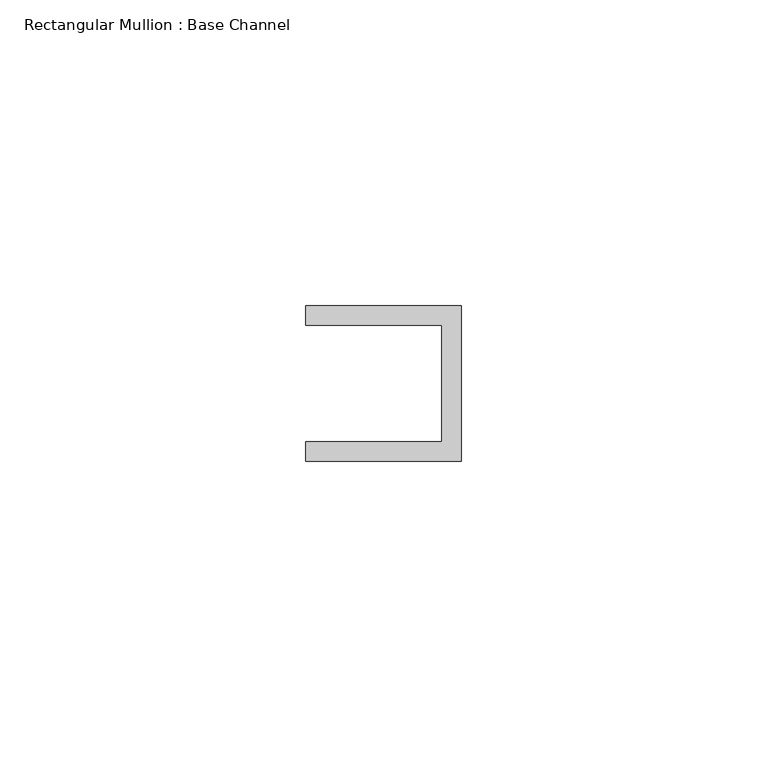
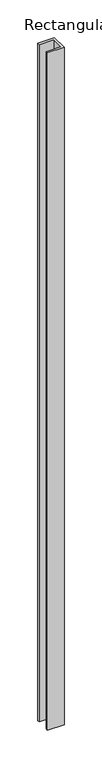
"""IFC4 building model written with IfcOpenShell, lengths in millimetres: member geometry, Rectangular Mullion : Base Channel."""

from ifc_helpers import new_model, si_unit, frame, origin, place, context, project, spatial, polyline, outline, extrude, source, transform, mapped, element, save


def rectangular_mullion_base_channel_b9c382ca(model_context):
    return source(origin(), model_context, "Body", "SweptSolid", [
        extrude(outline(polyline([(0.0, -12.7), (-25.4, -12.7), (-25.4, -9.525), (-3.175, -9.525), (-3.175, 9.525), (-25.4, 9.525), (-25.4, 12.7), (0.0, 12.7), (0.0, -12.7)])), frame((0.0, 0.0, -1092.2), z_axis=(0.0, 0.0, 1.0), x_axis=(1.0, 0.0, 0.0)), (0.0, 0.0, 1.0), 1092.2),
    ])


if __name__ == "__main__":
    model = new_model("IFC4")
    model_context = context("Model", 3, world=origin())
    ifc_project = project(units=[si_unit("LENGTHUNIT", "METRE", prefix="MILLI")], contexts=[model_context])
    site = spatial("IfcSite", under=ifc_project)
    building = spatial("IfcBuilding", under=site)
    placement = place(None, origin())
    rectangular_mullion_base_channel_shape = rectangular_mullion_base_channel_b9c382ca(model_context)
    element("IfcMember", 1, ObjectType="Rectangular Mullion : Base Channel", at=placement, inside=building, context=model_context, shape_type="MappedRepresentation", body=[
        mapped(rectangular_mullion_base_channel_shape, transform((0.0, 0.0, 0.0), x_axis=(1.0, 0.0, 0.0), y_axis=(0.0, 1.0, 0.0), z_axis=(0.0, 0.0, 1.0))),
    ])
    save(model, "model.ifc")

# Revit data of these elements
# Type "Rectangular Mullion : Base Channel"
#   built-in parameter 1007322 = 0.0833333 (stored number, unit not read)
#   built-in parameter 1007321 = 0.0416667 (stored number, unit not read)
#   built-in parameter 1007320 = -0.03125 (stored number, unit not read)
# Element 1 (IfcMember, "Rectangular Mullion : Base Channel")
#   Materials on its faces: "ALUM"
# Materials
#   "ALUM": class "Generic", colour RGB 157 157 157, transparency 0, Cost = 0
